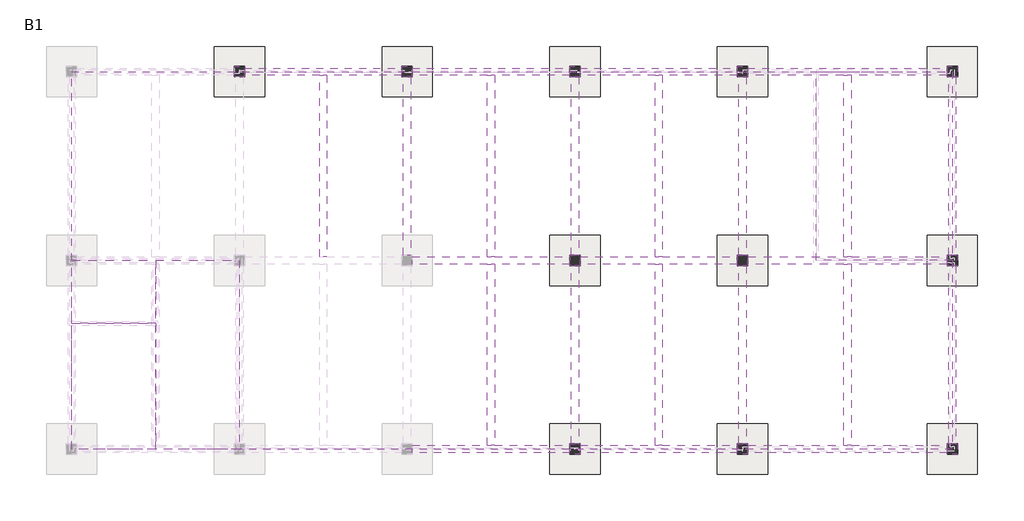
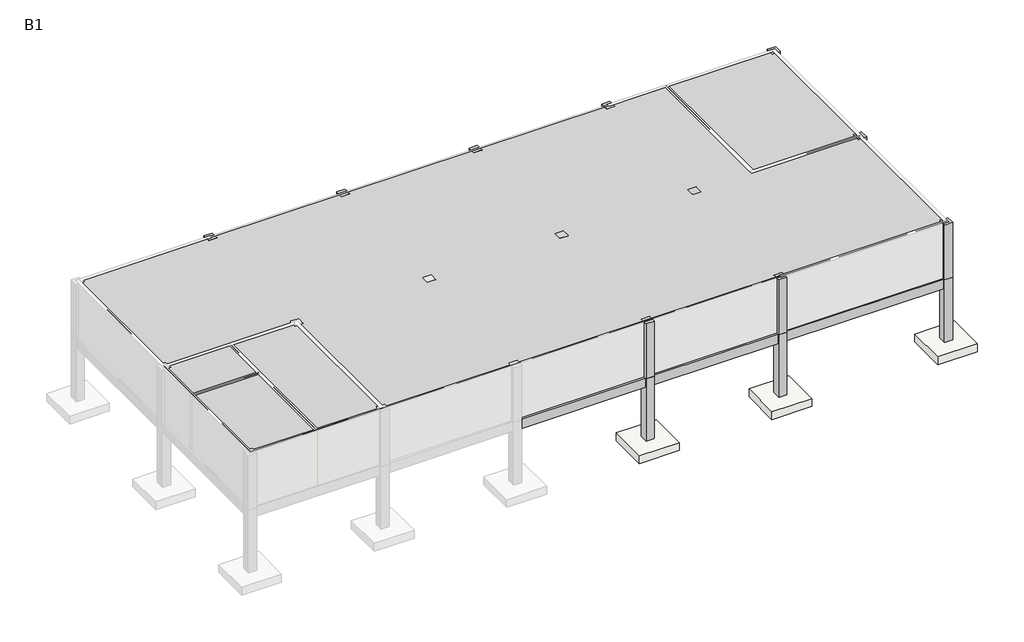
# One storey, part 2 of 2: 24 beams, 22 columns, 11 slabs, 5 proxies.
# Revit data of these elements (continued)
# Element 25 (IfcBuildingElementProxy, "Space Planning Box_hec : Space Planning Box_hec") (continued)
#   Exterior Finish = "N/A..N/A,,EW1..EW2..N/A"
#   Department = "EL"
#   ceiling height = 0
#   Width = 18000 mm
#   Program Area = 720.00 m²
#   Length = 42000 mm
#   Height = 3500 mm
#   Area = 756.00 m²
#   Fill Color = Orange
#   Phase Created = New Construction
#   Materials on its faces: "Orange"
# Element 26 (IfcBuildingElementProxy, "Space Planning Box_hec : Space Planning Box_hec")
#   Room Name = "Battery Room"
#   Interior Finish = "IW2..N/A..N/A,,N/A..N/A,,FL7..N/A,,CL2..N/A"
#   Exterior Finish = "N/A..N/A,,EW2..N/A..N/A"
#   Department = "EL"
#   ceiling height = 0
#   Width = 6500 mm
#   Program Area = 58.50 m²
#   Length = 9000 mm
#   Height = 3500 mm
#   Area = 58.50 m²
#   Fill Color = Orange
#   Phase Created = New Construction
#   Materials on its faces: "Orange"
# Element 27 (IfcBuildingElementProxy, "Space Planning Box_hec : Space Planning Box_hec")
#   Room Name = "Lobby"
#   Interior Finish = "IW5..N/A..N/A,,WK3..N/A,,FL2..N/A,,N/A..N/A"
#   Exterior Finish = "N/A..N/A,,EW2..N/A..N/A"
#   Department = "AR"
#   ceiling height = 0
#   Width = 4000 mm
#   Program Area = 0.00 m²
#   Length = 9000 mm
#   Height = 3500 mm
#   Area = 36.00 m²
#   Fill Color = Cyan
#   Phase Created = New Construction
#   Materials on its faces: "Cyan"
# Element 28 (IfcBuildingElementProxy, "Space Planning Box_hec : Space Planning Box_hec")
#   Room Name = "Elevator"
#   Interior Finish = "N/A..N/A..N/A,,N/A..N/A,,,,CL3..N/A"
#   Exterior Finish = "N/A..N/A,,EW2..N/A..N/A"
#   Department = "AR"
#   ceiling height = 0
#   Width = 4000 mm
#   Program Area = 0.00 m²
#   Length = 3000 mm
#   Height = 3500 mm
#   Area = 12.00 m²
#   Fill Color = Cyan
#   Phase Created = New Construction
#   Materials on its faces: "Cyan"
# Element 29 (IfcBuildingElementProxy, "Space Planning Box_hec : Space Planning Box_hec")
#   Room Name = "Stairway"
#   Interior Finish = "IW5..N/A..N/A,,WK3..N/A,,FL2..N/A,,CL1..N/A"
#   Exterior Finish = "N/A..N/A,,EW2..N/A..N/A"
#   Department = "PATHV1"
#   ceiling height = 0
#   Width = 4000 mm
#   Program Area = 36.00 m²
#   Length = 6000 mm
#   Height = 3500 mm
#   Area = 24.00 m²
#   Fill Color = Green
#   Phase Created = New Construction
#   Materials on its faces: "Green"
# Elements 30, 31, 32, 33, 34, 35, 36, 37, 38, 39, 40, 41, 42, 43, 44, 45, 46, 47, 48, 49, 50, 51 (IfcColumn, "Concrete-Rectangular-Column : CL111_500x500")
#   Comments = ""
#   hec_material3 = none
#   hec_material2 = none
#   hec_material1 = none
#   Structural Material = 콘크리트 - 현장타설 콘크리트
#   Phase Created = New Construction
#   Materials on its faces: "콘크리트 - 현장타설 콘크리트"
# Elements 52, 53, 54, 55, 56, 57, 58, 59, 60, 61, 62 (IfcSlab, "FT112-Footing-Rectangular : FT112_2400x2400x500")
#   Comments = ""
#   hec_material3 = none
#   hec_material2 = none
#   hec_material1 = none
#   Structural Material = 콘크리트 - 현장타설 콘크리트
#   Phase Created = New Construction
#   Materials on its faces: "콘크리트 - 현장타설 콘크리트"
# Materials
#   "콘크리트 - 현장타설 콘크리트": class "콘크리트", colour RGB 192 192 192, transparency 0
#   "Cyan": class "Generic", colour RGB 0 255 255, transparency 0.2, Cost = 0
#   "A03AE056-00001_Bitumen/Bituminous/Asphalt Coating": class "Generic", colour RGB 17 17 17, transparency 0, Description = "Damp-proofing", W00) Work Master Code = "A03AE056-00001", W01) Work Master_Lv1 = "Concrete Work", W02) Work Master_Lv2 = "Concrete Protective Coating (U/G)", W03) Work Master_Spec.1 = "Bitumen/Bituminous/Asphalt Coating", Cost = 0
#   "A03AC035-00001_Form Work (3 times in use)_Flat": class "Wood", colour RGB 149 120 74, transparency 0, Description = "Plywood", W00) Work Master Code = "A03AC035-00001", W01) Work Master_Lv1 = "Concrete Work", W02) Work Master_Lv2 = "Substructure Work", W03) Work Master_Spec.1 = "Form Work (3 times in use)", W04) Work Master_Spec.2 = "Flat Form", W05) Work Master_Spec.3 = "Dressed Lumber, Plywood or Steel Form(Wood Planks are not Allowed) incl. Chamfer", Cost = 0
#   "A03AC032-00007_Structural Concrete_Type1_25MPa-30Mpa": class "Concrete", colour RGB 176 176 176, transparency 0, Keynote = "09910.A1", Description = "Reinf. Conc.", W00) Work Master Code = "A03AC032-00007", W01) Work Master_Lv1 = "Concrete Work", W02) Work Master_Lv2 = "Substructure Work", W03) Work Master_Spec.1 = "Structural Concrete", W04) Work Master_Spec.2 = "Cement Type-1", W05) Work Master_Spec.3 = "25MPa < F'c (Cylinder Strength) ≤ 30MPa", Cost = 0
#   "Orange": class "Generic", colour RGB 255 165 0, transparency 0.2, Cost = 0
#   "Green": class "Generic", colour RGB 0 128 0, transparency 0.2, Cost = 0
